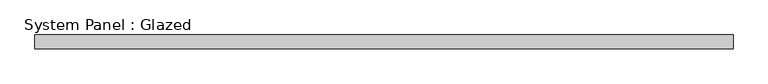
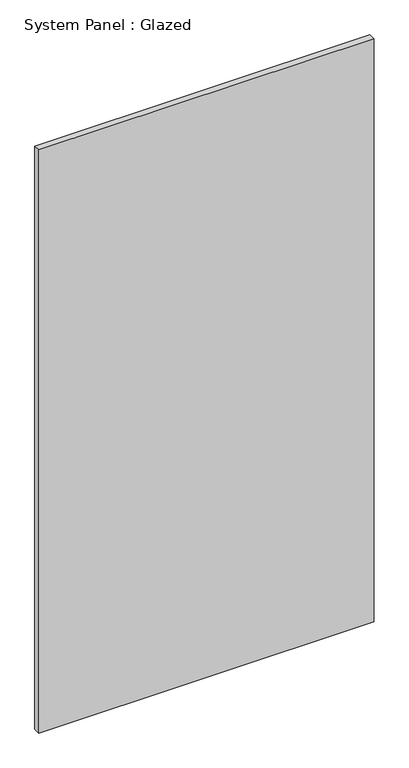
"""IFC4 building model written with IfcOpenShell, lengths in millimetres: plate geometry, System Panel : Glazed."""

import ifcopenshell
import ifcopenshell.guid

model = None  # the IFC model being written
_history = None  # IfcOwnerHistory: only IFC2X3 demands one
_inside = {}  # id of a spatial element -> (the spatial element, [elements in it])
_under = {}  # id of a project, library or spatial element -> (it, [spatial elements below it])
_declared = {}  # id of a project -> (the project, [libraries it declares])
_typed = {}  # id of a type object -> (the type object, [elements of that type])
_made_of = {}  # id of a material, layer set ... -> (it, [elements and type objects made of it])


def new_model(schema):
    """Start an empty IFC model of exactly this schema.

    Asked for "IFC4X3", IfcOpenShell would pick the latest addendum, in which some entities
    have other attributes; the version numbers below select the first issue.
    IFC2X3 requires an IfcOwnerHistory on every rooted entity: one is made here for all.
    """
    global model, _history
    if schema == "IFC4X3":
        model = ifcopenshell.file(schema_version=(4, 3, 0, 0))
    else:
        model = ifcopenshell.file(schema=schema)
    _inside.clear()
    _under.clear()
    _declared.clear()
    _typed.clear()
    _made_of.clear()
    _history = None
    if model.schema == "IFC2X3":
        org = make("IfcOrganization", Name="unknown")
        user = make(
            "IfcPersonAndOrganization",
            ThePerson=make("IfcPerson", FamilyName="unknown"),
            TheOrganization=org,
        )
        app = make(
            "IfcApplication",
            ApplicationDeveloper=org,
            Version="unknown",
            ApplicationFullName="unknown",
            ApplicationIdentifier="unknown",
        )
        _history = make(
            "IfcOwnerHistory",
            OwningUser=user,
            OwningApplication=app,
            ChangeAction="ADDED",
            CreationDate=0,
        )
    return model


def make(cls, **values):
    """One entity of the class cls with the attributes given. An attribute that is None is left unset."""
    return model.create_entity(
        cls, **{name: value for name, value in values.items() if value is not None}
    )


def rooted(cls, **values):
    """An entity with a GlobalId (a new one), such as an element, a storey or a relation."""
    return make(cls, GlobalId=ifcopenshell.guid.new(), OwnerHistory=_history, **values)


def si_unit(unit_type, name, prefix=None):
    """IfcSIUnit, for example si_unit("LENGTHUNIT", "METRE", prefix="MILLI")."""
    return make("IfcSIUnit", UnitType=unit_type, Prefix=prefix, Name=name)


def assignment(units):
    """IfcUnitAssignment: the units of a project."""
    return None if units is None else make("IfcUnitAssignment", Units=units)


def point(xyz):
    """IfcCartesianPoint."""
    return None if xyz is None else make("IfcCartesianPoint", Coordinates=xyz)


def direction(xyz):
    """IfcDirection."""
    return None if xyz is None else make("IfcDirection", DirectionRatios=xyz)


def frame(location, z_axis=None, x_axis=None):
    """IfcAxis2Placement3D, a coordinate frame: its origin and axes. An axis left out is left unset."""
    return make(
        "IfcAxis2Placement3D",
        Location=point(location),
        Axis=direction(z_axis),
        RefDirection=direction(x_axis),
    )


def origin():
    """The frame at (0, 0, 0) with its axes left unset."""
    return frame((0.0, 0.0, 0.0))


def origin_with_axes():
    """The frame at (0, 0, 0) with the z axis (0, 0, 1) and the x axis (1, 0, 0) written out."""
    return frame((0.0, 0.0, 0.0), z_axis=(0.0, 0.0, 1.0), x_axis=(1.0, 0.0, 0.0))


def place(relative_to, where):
    """IfcLocalPlacement: puts the frame where relative to a parent placement (None: the world)."""
    return make(
        "IfcLocalPlacement", PlacementRelTo=relative_to, RelativePlacement=where
    )


def context(
    kind, dimensions, precision=None, world=None, true_north=None, identifier=None
):
    """IfcGeometricRepresentationContext, for example the 3D "Model" context."""
    return make(
        "IfcGeometricRepresentationContext",
        ContextIdentifier=identifier,
        ContextType=kind,
        CoordinateSpaceDimension=dimensions,
        Precision=precision,
        WorldCoordinateSystem=world,
        TrueNorth=true_north,
    )


def project(units=None, contexts=None):
    """IfcProject with its units and contexts."""
    return rooted(
        "IfcProject",
        Name="project",
        RepresentationContexts=contexts,
        UnitsInContext=assignment(units),
    )


def spatial(cls, under=None, at=None, **own):
    """A site, building, storey or space (cls), placed at a placement, below another one or the project."""
    s = rooted(cls, ObjectPlacement=at, **own)
    if under is not None:
        _under.setdefault(under.id(), (under, []))[1].append(s)
    return s


def polyline(points):
    """IfcPolyline through the points."""
    return make("IfcPolyline", Points=[point(p) for p in points])


def outline(outer, holes=None, kind="AREA"):
    """IfcArbitraryClosedProfileDef: a profile drawn as a closed curve; with holes, ...WithVoids."""
    if holes is None:
        return make("IfcArbitraryClosedProfileDef", ProfileType=kind, OuterCurve=outer)
    return make(
        "IfcArbitraryProfileDefWithVoids",
        ProfileType=kind,
        OuterCurve=outer,
        InnerCurves=holes,
    )


def extrude(swept, where, along, depth):
    """IfcExtrudedAreaSolid: the profile swept, set in the frame where, extruded along a direction by depth."""
    return make(
        "IfcExtrudedAreaSolid",
        SweptArea=swept,
        Position=where,
        ExtrudedDirection=direction(along),
        Depth=depth,
    )


def shape(context_of_items, identifier, shape_type, items):
    """IfcShapeRepresentation: the items that make up one representation, for example the "Body"."""
    return make(
        "IfcShapeRepresentation",
        ContextOfItems=context_of_items,
        RepresentationIdentifier=identifier,
        RepresentationType=shape_type,
        Items=items,
    )


def source(mapping_origin, context_of_items, identifier, shape_type, items):
    """IfcRepresentationMap: a shape defined once, which mapped items show again and again."""
    return make(
        "IfcRepresentationMap",
        MappingOrigin=mapping_origin,
        MappedRepresentation=shape(context_of_items, identifier, shape_type, items),
    )


def transform(
    local_origin,
    x_axis=None,
    y_axis=None,
    z_axis=None,
    scale=None,
    scale2=None,
    scale3=None,
    uniform=True,
):
    """IfcCartesianTransformationOperator3D, or its non-uniform kind. x_axis, y_axis, z_axis: its Axis1, 2, 3."""
    if uniform:
        return make(
            "IfcCartesianTransformationOperator3D",
            Axis1=direction(x_axis),
            Axis2=direction(y_axis),
            LocalOrigin=point(local_origin),
            Scale=scale,
            Axis3=direction(z_axis),
        )
    return make(
        "IfcCartesianTransformationOperator3DnonUniform",
        Axis1=direction(x_axis),
        Axis2=direction(y_axis),
        LocalOrigin=point(local_origin),
        Scale=scale,
        Axis3=direction(z_axis),
        Scale2=scale2,
        Scale3=scale3,
    )


def mapped(mapping_source, mapping_target):
    """IfcMappedItem: shows the shape of a source again, moved by a transform."""
    return make(
        "IfcMappedItem", MappingSource=mapping_source, MappingTarget=mapping_target
    )


def made_of(thing, what):
    """Note that an element or type object is made of a material, layer set ...; save() writes the relation."""
    if what is not None:
        _made_of.setdefault(what.id(), (what, []))[1].append(thing)
    return thing


def element(
    cls,
    number,
    at=None,
    inside=None,
    cuts=None,
    type_object=None,
    material=None,
    context=None,
    identifier="Body",
    shape_type=None,
    held_by="IfcProductDefinitionShape",
    body=None,
    shapes=None,
    **own,
):
    """One element of the class cls, such as IfcWall. Its Tag is "e" and its number.

    at: its placement. inside: the storey or other place that contains it. cuts: it is an
    opening in that element (IfcRelVoidsElement). A single representation is given by context,
    identifier, shape_type and body (its items); several are given by shapes. held_by: the class
    of the entity that holds the representations. save() writes the other relations.
    """
    e = rooted(cls, Tag="e%d" % number, ObjectPlacement=at, **own)
    if body is not None:
        shapes = [shape(context, identifier, shape_type, body)]
    if shapes is not None:
        e.Representation = make(held_by, Representations=shapes)
    if inside is not None:
        _inside.setdefault(inside.id(), (inside, []))[1].append(e)
    if cuts is not None:
        rooted(
            "IfcRelVoidsElement", RelatingBuildingElement=cuts, RelatedOpeningElement=e
        )
    if type_object is not None:
        _typed.setdefault(type_object.id(), (type_object, []))[1].append(e)
    return made_of(e, material)


def aggregate(whole, parts):
    """IfcRelAggregates: a whole, such as a stair, and the parts it consists of."""
    return rooted("IfcRelAggregates", RelatingObject=whole, RelatedObjects=parts)


def save(model, path):
    """Write the relations noted so far, then the file.

    IfcRelAggregates (storeys below a building ...), IfcRelContainedInSpatialStructure (elements
    in a storey), IfcRelDefinesByType, IfcRelAssociatesMaterial and IfcRelDeclares: one each for
    every whole, place, type object, material and project.
    """
    for whole, parts in _under.values():
        aggregate(whole, parts)
    for where, things in _inside.values():
        rooted(
            "IfcRelContainedInSpatialStructure",
            RelatedElements=things,
            RelatingStructure=where,
        )
    for kind, things in _typed.values():
        rooted("IfcRelDefinesByType", RelatedObjects=things, RelatingType=kind)
    for what, things in _made_of.values():
        rooted("IfcRelAssociatesMaterial", RelatedObjects=things, RelatingMaterial=what)
    for by, libraries in _declared.values():
        rooted("IfcRelDeclares", RelatingContext=by, RelatedDefinitions=libraries)
    model.write(path)


def system_panel_glazed_5b896d3e(model_context):
    return source(origin(), model_context, "Body", "SweptSolid", [
        extrude(outline(polyline([(639.2857142, 24.5), (-639.2857142, 24.5), (-639.2857142, 49.5), (639.2857142, 49.5), (639.2857142, 24.5)])), origin_with_axes(), (0.0, 0.0, 1.0), 2350.0),
    ])


if __name__ == "__main__":
    model = new_model("IFC4")
    model_context = context("Model", 3, world=origin())
    ifc_project = project(units=[si_unit("LENGTHUNIT", "METRE", prefix="MILLI")], contexts=[model_context])
    site = spatial("IfcSite", under=ifc_project)
    building = spatial("IfcBuilding", under=site)
    placement = place(None, origin())
    system_panel_glazed_shape = system_panel_glazed_5b896d3e(model_context)
    element("IfcPlate", 1, ObjectType="System Panel : Glazed", at=placement, inside=building, context=model_context, shape_type="MappedRepresentation", body=[
        mapped(system_panel_glazed_shape, transform((0.0, 0.0, 0.0), x_axis=(1.0, 0.0, 0.0), y_axis=(0.0, 1.0, 0.0), z_axis=(0.0, 0.0, 1.0))),
    ])
    save(model, "model.ifc")

# Revit data of these elements
# Type "System Panel : Glazed"
#   Construction Type Id = "GSP4R"
#   Analytic Construction = "1/8 in Pilkington single glazing"
#   Visual Light Transmittance = 0.9
#   Solar Heat Gain Coefficient = 0.86
#   Heat Transfer Coefficient (U) = 6.7069 W/(m²·K)
#   Define Thermal Properties by = 1
# Element 1 (IfcPlate, "System Panel : Glazed")
#   Materials on its faces: "Glass"
# Materials
#   "Glass": class "Glass", colour RGB 0 128 192, transparency 0.75, Description = "Soda Lime Glass", Cost = 0
